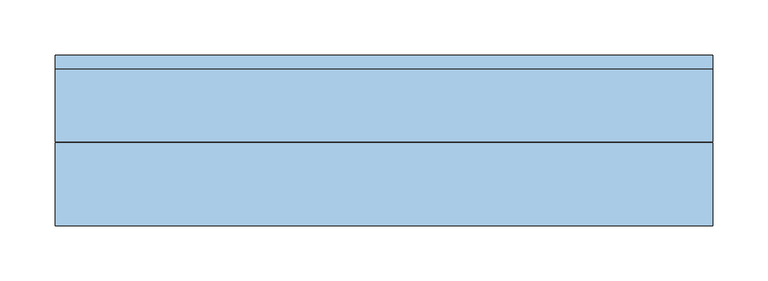
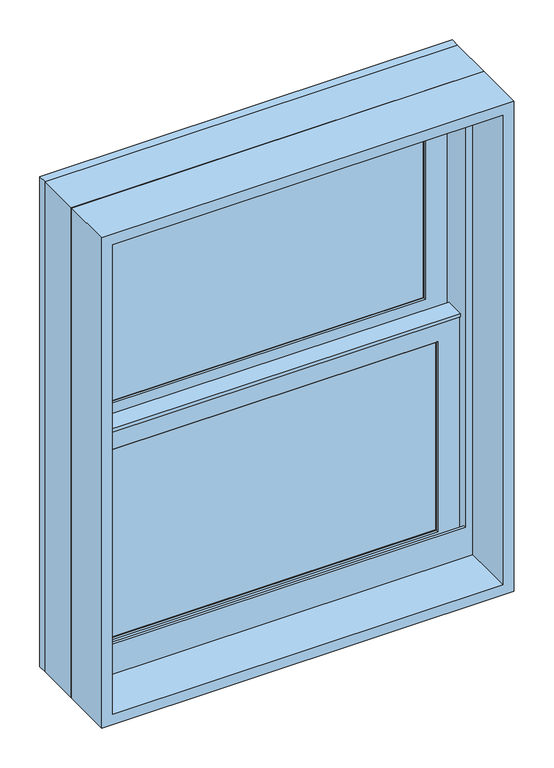
"""IFC4 building model written with IfcOpenShell, lengths in millimetres: window geometry, Window-Double_Hung-Marvin-Essential : ESDH2026."""

import ifcopenshell
import ifcopenshell.guid

model = None  # the IFC model being written
_history = None  # IfcOwnerHistory: only IFC2X3 demands one
_inside = {}  # id of a spatial element -> (the spatial element, [elements in it])
_under = {}  # id of a project, library or spatial element -> (it, [spatial elements below it])
_declared = {}  # id of a project -> (the project, [libraries it declares])
_typed = {}  # id of a type object -> (the type object, [elements of that type])
_made_of = {}  # id of a material, layer set ... -> (it, [elements and type objects made of it])


def new_model(schema):
    """Start an empty IFC model of exactly this schema.

    Asked for "IFC4X3", IfcOpenShell would pick the latest addendum, in which some entities
    have other attributes; the version numbers below select the first issue.
    IFC2X3 requires an IfcOwnerHistory on every rooted entity: one is made here for all.
    """
    global model, _history
    if schema == "IFC4X3":
        model = ifcopenshell.file(schema_version=(4, 3, 0, 0))
    else:
        model = ifcopenshell.file(schema=schema)
    _inside.clear()
    _under.clear()
    _declared.clear()
    _typed.clear()
    _made_of.clear()
    _history = None
    if model.schema == "IFC2X3":
        org = make("IfcOrganization", Name="unknown")
        user = make(
            "IfcPersonAndOrganization",
            ThePerson=make("IfcPerson", FamilyName="unknown"),
            TheOrganization=org,
        )
        app = make(
            "IfcApplication",
            ApplicationDeveloper=org,
            Version="unknown",
            ApplicationFullName="unknown",
            ApplicationIdentifier="unknown",
        )
        _history = make(
            "IfcOwnerHistory",
            OwningUser=user,
            OwningApplication=app,
            ChangeAction="ADDED",
            CreationDate=0,
        )
    return model


def make(cls, **values):
    """One entity of the class cls with the attributes given. An attribute that is None is left unset."""
    return model.create_entity(
        cls, **{name: value for name, value in values.items() if value is not None}
    )


def rooted(cls, **values):
    """An entity with a GlobalId (a new one), such as an element, a storey or a relation."""
    return make(cls, GlobalId=ifcopenshell.guid.new(), OwnerHistory=_history, **values)


def si_unit(unit_type, name, prefix=None):
    """IfcSIUnit, for example si_unit("LENGTHUNIT", "METRE", prefix="MILLI")."""
    return make("IfcSIUnit", UnitType=unit_type, Prefix=prefix, Name=name)


def assignment(units):
    """IfcUnitAssignment: the units of a project."""
    return None if units is None else make("IfcUnitAssignment", Units=units)


def point(xyz):
    """IfcCartesianPoint."""
    return None if xyz is None else make("IfcCartesianPoint", Coordinates=xyz)


def direction(xyz):
    """IfcDirection."""
    return None if xyz is None else make("IfcDirection", DirectionRatios=xyz)


def frame(location, z_axis=None, x_axis=None):
    """IfcAxis2Placement3D, a coordinate frame: its origin and axes. An axis left out is left unset."""
    return make(
        "IfcAxis2Placement3D",
        Location=point(location),
        Axis=direction(z_axis),
        RefDirection=direction(x_axis),
    )


def origin():
    """The frame at (0, 0, 0) with its axes left unset."""
    return frame((0.0, 0.0, 0.0))


def place(relative_to, where):
    """IfcLocalPlacement: puts the frame where relative to a parent placement (None: the world)."""
    return make(
        "IfcLocalPlacement", PlacementRelTo=relative_to, RelativePlacement=where
    )


def context(
    kind, dimensions, precision=None, world=None, true_north=None, identifier=None
):
    """IfcGeometricRepresentationContext, for example the 3D "Model" context."""
    return make(
        "IfcGeometricRepresentationContext",
        ContextIdentifier=identifier,
        ContextType=kind,
        CoordinateSpaceDimension=dimensions,
        Precision=precision,
        WorldCoordinateSystem=world,
        TrueNorth=true_north,
    )


def project(units=None, contexts=None):
    """IfcProject with its units and contexts."""
    return rooted(
        "IfcProject",
        Name="project",
        RepresentationContexts=contexts,
        UnitsInContext=assignment(units),
    )


def spatial(cls, under=None, at=None, **own):
    """A site, building, storey or space (cls), placed at a placement, below another one or the project."""
    s = rooted(cls, ObjectPlacement=at, **own)
    if under is not None:
        _under.setdefault(under.id(), (under, []))[1].append(s)
    return s


def polyline(points):
    """IfcPolyline through the points."""
    return make("IfcPolyline", Points=[point(p) for p in points])


def outline(outer, holes=None, kind="AREA"):
    """IfcArbitraryClosedProfileDef: a profile drawn as a closed curve; with holes, ...WithVoids."""
    if holes is None:
        return make("IfcArbitraryClosedProfileDef", ProfileType=kind, OuterCurve=outer)
    return make(
        "IfcArbitraryProfileDefWithVoids",
        ProfileType=kind,
        OuterCurve=outer,
        InnerCurves=holes,
    )


def extrude(swept, where, along, depth):
    """IfcExtrudedAreaSolid: the profile swept, set in the frame where, extruded along a direction by depth."""
    return make(
        "IfcExtrudedAreaSolid",
        SweptArea=swept,
        Position=where,
        ExtrudedDirection=direction(along),
        Depth=depth,
    )


def faces_of(points, faces, orient=None, outer=None):
    """IfcFace entities. A face is a list of loops; a loop is a list of indices into points, from 0.

    orient and outer hold one flag for each loop. By default every Orientation is true, the
    first loop of a face is its IfcFaceOuterBound and the others are IfcFaceBound.
    """
    made = []
    for i, loops in enumerate(faces):
        bounds = []
        for j, loop in enumerate(loops):
            is_outer = j == 0 if outer is None else outer[i][j]
            bounds.append(
                make(
                    "IfcFaceOuterBound" if is_outer else "IfcFaceBound",
                    Bound=make("IfcPolyLoop", Polygon=[points[k] for k in loop]),
                    Orientation=True if orient is None else orient[i][j],
                )
            )
        made.append(make("IfcFace", Bounds=bounds))
    return made


def faceted_brep(points, faces, orient=None, outer=None, voids=None):
    """IfcFacetedBrep: a solid bounded by flat faces; with voids (closed shells), ...WithVoids."""
    shared = [point(p) for p in points]
    hull = make("IfcClosedShell", CfsFaces=faces_of(shared, faces, orient, outer))
    if voids is None:
        return make("IfcFacetedBrep", Outer=hull)
    return make(
        "IfcFacetedBrepWithVoids",
        Outer=hull,
        Voids=[
            make(cls, CfsFaces=faces_of(shared, fs, o, b)) for cls, fs, o, b in voids
        ],
    )


def shape(context_of_items, identifier, shape_type, items):
    """IfcShapeRepresentation: the items that make up one representation, for example the "Body"."""
    return make(
        "IfcShapeRepresentation",
        ContextOfItems=context_of_items,
        RepresentationIdentifier=identifier,
        RepresentationType=shape_type,
        Items=items,
    )


def source(mapping_origin, context_of_items, identifier, shape_type, items):
    """IfcRepresentationMap: a shape defined once, which mapped items show again and again."""
    return make(
        "IfcRepresentationMap",
        MappingOrigin=mapping_origin,
        MappedRepresentation=shape(context_of_items, identifier, shape_type, items),
    )


def transform(
    local_origin,
    x_axis=None,
    y_axis=None,
    z_axis=None,
    scale=None,
    scale2=None,
    scale3=None,
    uniform=True,
):
    """IfcCartesianTransformationOperator3D, or its non-uniform kind. x_axis, y_axis, z_axis: its Axis1, 2, 3."""
    if uniform:
        return make(
            "IfcCartesianTransformationOperator3D",
            Axis1=direction(x_axis),
            Axis2=direction(y_axis),
            LocalOrigin=point(local_origin),
            Scale=scale,
            Axis3=direction(z_axis),
        )
    return make(
        "IfcCartesianTransformationOperator3DnonUniform",
        Axis1=direction(x_axis),
        Axis2=direction(y_axis),
        LocalOrigin=point(local_origin),
        Scale=scale,
        Axis3=direction(z_axis),
        Scale2=scale2,
        Scale3=scale3,
    )


def mapped(mapping_source, mapping_target):
    """IfcMappedItem: shows the shape of a source again, moved by a transform."""
    return make(
        "IfcMappedItem", MappingSource=mapping_source, MappingTarget=mapping_target
    )


def made_of(thing, what):
    """Note that an element or type object is made of a material, layer set ...; save() writes the relation."""
    if what is not None:
        _made_of.setdefault(what.id(), (what, []))[1].append(thing)
    return thing


def element(
    cls,
    number,
    at=None,
    inside=None,
    cuts=None,
    type_object=None,
    material=None,
    context=None,
    identifier="Body",
    shape_type=None,
    held_by="IfcProductDefinitionShape",
    body=None,
    shapes=None,
    **own,
):
    """One element of the class cls, such as IfcWall. Its Tag is "e" and its number.

    at: its placement. inside: the storey or other place that contains it. cuts: it is an
    opening in that element (IfcRelVoidsElement). A single representation is given by context,
    identifier, shape_type and body (its items); several are given by shapes. held_by: the class
    of the entity that holds the representations. save() writes the other relations.
    """
    e = rooted(cls, Tag="e%d" % number, ObjectPlacement=at, **own)
    if body is not None:
        shapes = [shape(context, identifier, shape_type, body)]
    if shapes is not None:
        e.Representation = make(held_by, Representations=shapes)
    if inside is not None:
        _inside.setdefault(inside.id(), (inside, []))[1].append(e)
    if cuts is not None:
        rooted(
            "IfcRelVoidsElement", RelatingBuildingElement=cuts, RelatedOpeningElement=e
        )
    if type_object is not None:
        _typed.setdefault(type_object.id(), (type_object, []))[1].append(e)
    return made_of(e, material)


def aggregate(whole, parts):
    """IfcRelAggregates: a whole, such as a stair, and the parts it consists of."""
    return rooted("IfcRelAggregates", RelatingObject=whole, RelatedObjects=parts)


def save(model, path):
    """Write the relations noted so far, then the file.

    IfcRelAggregates (storeys below a building ...), IfcRelContainedInSpatialStructure (elements
    in a storey), IfcRelDefinesByType, IfcRelAssociatesMaterial and IfcRelDeclares: one each for
    every whole, place, type object, material and project.
    """
    for whole, parts in _under.values():
        aggregate(whole, parts)
    for where, things in _inside.values():
        rooted(
            "IfcRelContainedInSpatialStructure",
            RelatedElements=things,
            RelatingStructure=where,
        )
    for kind, things in _typed.values():
        rooted("IfcRelDefinesByType", RelatedObjects=things, RelatingType=kind)
    for what, things in _made_of.values():
        rooted("IfcRelAssociatesMaterial", RelatedObjects=things, RelatingMaterial=what)
    for by, libraries in _declared.values():
        rooted("IfcRelDeclares", RelatingContext=by, RelatedDefinitions=libraries)
    model.write(path)


def window_7cff9b80(model_context):
    return source(origin(), model_context, "Body", "SolidModel", [
        extrude(outline(polyline([(89.9583333, 20.6375), (89.9583333, 15.875), (70.9083333, 15.875), (70.9083333, 20.6375), (89.9583333, 20.6375)])), frame((0.0, 0.0, 1746.25), z_axis=(0.0, 0.0, 1.0), x_axis=(1.0, 0.0, 0.0)), (0.0, 0.0, 1.0), 298.45),
        extrude(outline(polyline([(-70.9083333, 20.6375), (-70.9083333, 15.875), (-89.9583333, 15.875), (-89.9583333, 20.6375), (-70.9083333, 20.6375)])), frame((0.0, 0.0, 1746.25), z_axis=(0.0, 0.0, 1.0), x_axis=(1.0, 0.0, 0.0)), (0.0, 0.0, 1.0), 298.45),
        extrude(outline(polyline([(241.3, 20.6375), (241.3, 15.875), (-241.3, 15.875), (-241.3, 20.6375), (241.3, 20.6375)])), frame((0.0, 0.0, 1885.95), z_axis=(0.0, 0.0, 1.0), x_axis=(1.0, 0.0, 0.0)), (0.0, 0.0, 1.0), 19.05),
        extrude(outline(polyline([(-89.9583333, 46.83125), (-89.9583333, 51.59375), (-70.9083333, 51.59375), (-70.9083333, 46.83125), (-89.9583333, 46.83125)])), frame((0.0, 0.0, 2082.8), z_axis=(0.0, 0.0, 1.0), x_axis=(1.0, 0.0, 0.0)), (0.0, 0.0, 1.0), 298.45),
        extrude(outline(polyline([(70.9083333, 46.83125), (70.9083333, 51.59375), (89.9583333, 51.59375), (89.9583333, 46.83125), (70.9083333, 46.83125)])), frame((0.0, 0.0, 2082.8), z_axis=(0.0, 0.0, 1.0), x_axis=(1.0, 0.0, 0.0)), (0.0, 0.0, 1.0), 298.45),
        extrude(outline(polyline([(-241.3, 46.83125), (-241.3, 51.59375), (241.3, 51.59375), (241.3, 46.83125), (-241.3, 46.83125)])), frame((0.0, 0.0, 2222.5), z_axis=(0.0, 0.0, 1.0), x_axis=(1.0, 0.0, 0.0)), (0.0, 0.0, 1.0), 19.05),
        extrude(outline(polyline([(89.9583333, 20.6375), (70.9083333, 20.6375), (70.9083333, 25.4), (89.9583333, 25.4), (89.9583333, 20.6375)])), frame((0.0, 0.0, 1746.25), z_axis=(0.0, 0.0, 1.0), x_axis=(1.0, 0.0, 0.0)), (0.0, 0.0, 1.0), 298.45),
        extrude(outline(polyline([(-70.9083333, 20.6375), (-89.9583333, 20.6375), (-89.9583333, 25.4), (-70.9083333, 25.4), (-70.9083333, 20.6375)])), frame((0.0, 0.0, 1746.25), z_axis=(0.0, 0.0, 1.0), x_axis=(1.0, 0.0, 0.0)), (0.0, 0.0, 1.0), 298.45),
        extrude(outline(polyline([(241.3, 20.6375), (-241.3, 20.6375), (-241.3, 25.4), (241.3, 25.4), (241.3, 20.6375)])), frame((0.0, 0.0, 1885.95), z_axis=(0.0, 0.0, 1.0), x_axis=(1.0, 0.0, 0.0)), (0.0, 0.0, 1.0), 19.05),
        extrude(outline(polyline([(-89.9583333, 56.35625), (-70.9083333, 56.35625), (-70.9083333, 51.59375), (-89.9583333, 51.59375), (-89.9583333, 56.35625)])), frame((0.0, 0.0, 2082.8), z_axis=(0.0, 0.0, 1.0), x_axis=(1.0, 0.0, 0.0)), (0.0, 0.0, 1.0), 298.45),
        extrude(outline(polyline([(70.9083333, 56.35625), (89.9583333, 56.35625), (89.9583333, 51.59375), (70.9083333, 51.59375), (70.9083333, 56.35625)])), frame((0.0, 0.0, 2082.8), z_axis=(0.0, 0.0, 1.0), x_axis=(1.0, 0.0, 0.0)), (0.0, 0.0, 1.0), 298.45),
        extrude(outline(polyline([(-241.3, 56.35625), (241.3, 56.35625), (241.3, 51.59375), (-241.3, 51.59375), (-241.3, 56.35625)])), frame((0.0, 0.0, 2222.5), z_axis=(0.0, 0.0, 1.0), x_axis=(1.0, 0.0, 0.0)), (0.0, 0.0, 1.0), 19.05),
        faceted_brep([(-268.2875, 5.6780605, 2074.7351748), (-268.2875, 5.6780605, 2070.1), (268.2875, 5.6780605, 2070.1), (268.2875, 5.6780605, 2074.7351748), (-268.2875, 34.8118605, 2074.7351748), (268.2875, 34.8118605, 2074.7351748), (268.2875, 34.8118605, 2070.1), (-268.2875, 34.8118605, 2070.1), (-268.2875, 30.1625, 2070.1), (-268.2875, 30.1625, 1719.2625), (-268.2875, 8.9241104, 1719.2625), (-268.2875, 8.9241104, 2070.1), (268.2875, 8.9241104, 2070.1), (268.2875, 30.1625, 2070.1), (268.2875, 8.9241104, 1719.2625), (268.2875, 30.1625, 1719.2625), (-252.4034752, 11.90625, 2055.8034752), (-252.4034752, 30.1625, 2055.8034752), (252.4034752, 30.1625, 2055.8034752), (252.4034752, 11.90625, 2055.8034752), (-235.74375, 10.4662439, 2039.14375), (-235.74375, 11.90625, 2039.14375), (235.74375, 11.90625, 2039.14375), (235.74375, 10.4662439, 2039.14375), (237.2858834, 8.9241104, 2040.6858834), (-237.2858834, 8.9241104, 2040.6858834), (252.4034752, 30.1625, 1735.1465248), (252.4034752, 11.90625, 1735.1465248), (235.74375, 11.90625, 1751.80625), (235.74375, 10.4662439, 1751.80625), (237.2858834, 8.9241104, 1750.2641166), (-252.4034752, 30.1625, 1735.1465248), (-252.4034752, 11.90625, 1735.1465248), (-235.74375, 11.90625, 1751.80625), (-235.74375, 10.4662439, 1751.80625), (-237.2858834, 8.9241104, 1750.2641166)], [[[0, 1, 2, 3]], [[4, 5, 6, 7]], [[1, 0, 4, 7, 8, 9, 10, 11]], [[2, 1, 11, 12]], [[7, 6, 13, 8]], [[3, 2, 12, 14, 15, 13, 6, 5]], [[0, 3, 5, 4]], [[16, 17, 18, 19]], [[20, 21, 22, 23]], [[20, 23, 24, 25]], [[19, 18, 26, 27]], [[23, 22, 28, 29]], [[24, 23, 29, 30]], [[27, 26, 31, 32]], [[29, 28, 33, 34]], [[30, 29, 34, 35]], [[15, 14, 10, 9]], [[15, 9, 8, 13], [18, 17, 31, 26]], [[17, 16, 32, 31]], [[16, 19, 27, 32], [22, 21, 33, 28]], [[21, 20, 34, 33]], [[20, 25, 35, 34]], [[10, 14, 12, 11], [25, 24, 30, 35]]]),
        extrude(outline(polyline([(38.5955581, 2055.8125), (33.5778968, 2055.8125), (33.5778968, 2057.4), (39.9405976, 2057.4), (39.9405976, 2055.8125), (61.515625, 2055.8125), (47.6307501, 2052.4975159), (38.5955581, 2052.4975159), (38.5955581, 2055.8125)])), frame((-268.2875, 0.0, 0.0), z_axis=(1.0, 0.0, 0.0), x_axis=(0.0, 1.0, 0.0)), (0.0, 0.0, 1.0), 536.575),
        faceted_brep([(298.45, 0.0, 1689.1), (298.45, 0.0, 2438.4), (-298.45, 0.0, 2438.4), (-298.45, 0.0, 1689.1), (272.25625, 0.0, 1750.21875), (-272.25625, 0.0, 1750.21875), (-272.25625, 0.0, 2412.20625), (272.25625, 0.0, 2412.20625), (272.25625, 3.96875, 1689.1), (-272.25625, 3.96875, 1689.1), (-272.25625, 3.96875, 1750.21875), (272.25625, 3.96875, 1750.21875), (-298.45, 65.6828125, 1689.1), (-272.25625, 65.6828125, 1689.1), (272.25625, 65.6828125, 1689.1), (298.45, 65.6828125, 1689.1), (-298.45, 65.6828125, 2438.4), (298.45, 65.6828125, 2438.4), (272.25625, 65.6828125, 2412.20625), (-272.25625, 65.6828125, 2412.20625)], [[[0, 1, 2, 3], [4, 5, 6, 7]], [[8, 9, 10, 11]], [[5, 4, 11, 10]], [[0, 3, 12, 13, 9, 8, 14, 15]], [[13, 12, 16, 17, 15, 14, 18, 19]], [[13, 19, 6, 5, 10, 9]], [[7, 6, 19, 18]], [[18, 14, 8, 11, 4, 7]], [[1, 0, 15, 17]], [[2, 1, 17, 16]], [[3, 2, 16, 12]]]),
        faceted_brep([(272.25625, 30.1625, 2063.75), (270.66875, 30.1625, 2063.75), (270.66875, 30.1625, 1713.4544613), (272.25625, 30.1625, 1713.4544613), (-270.66875, 30.1625, 2063.75), (-272.25625, 30.1625, 2063.75), (-272.25625, 30.1625, 1713.4544613), (-270.66875, 30.1625, 1713.4544613), (270.66875, 63.5, 2063.75), (272.25625, 63.5, 2063.75), (272.25625, 63.5, 1706.9743077), (270.66875, 63.5, 1706.9743077), (-272.25625, 63.5, 2063.75), (-270.66875, 63.5, 2063.75), (-270.66875, 63.5, 1706.9743077), (-272.25625, 63.5, 1706.9743077), (283.5108932, 3.96875, 1718.5460105), (283.5108932, 3.96875, 1689.1), (283.5108932, 65.6828125, 1689.1), (283.5108932, 65.6828125, 1706.550012), (-283.5108932, 3.96875, 1689.1), (-283.5108932, 3.96875, 1718.5460105), (-283.5108932, 65.6828125, 1706.550012), (-283.5108932, 65.6828125, 1689.1), (283.5108932, 78.58125, 1704.0428097), (-283.5108932, 78.58125, 1704.0428097), (-281.4971252, 68.2348864, 1706.0539391), (-263.53135, 68.2348864, 1706.0539391), (-263.53135, 65.6828125, 1706.550012), (263.53135, 65.6828125, 1706.550012), (263.53135, 68.2348864, 1706.0539391), (281.4971252, 68.2348864, 1706.0539391), (-298.45, 65.6828125, 1689.1), (-298.45, 78.5948249, 1689.1), (298.45, 78.5948249, 1689.1), (298.45, 65.6828125, 1689.1), (-298.45, 78.58125, 2438.4), (298.45, 78.58125, 2438.4), (283.5108932, 78.58125, 2423.4608932), (-283.5108932, 78.58125, 2423.4608932), (-298.45, 65.6828125, 2438.4), (-281.4971252, 68.2348864, 2421.4471252), (281.4971252, 68.2348864, 2421.4471252), (263.53135, 68.2348864, 2403.48135), (-263.53135, 68.2348864, 2403.48135), (-263.53135, 65.6828125, 2403.48135), (263.53135, 65.6828125, 2403.48135), (298.45, 65.6828125, 2438.4)], [[[0, 1, 2, 3]], [[4, 5, 6, 7]], [[8, 9, 10, 11]], [[12, 13, 14, 15]], [[1, 8, 11, 2]], [[9, 0, 3, 10]], [[1, 0, 9, 8]], [[5, 4, 13, 12]], [[5, 12, 15, 6]], [[13, 4, 7, 14]], [[16, 17, 18, 19]], [[20, 21, 22, 23]], [[24, 25, 26, 27, 28, 22, 21, 16, 19, 29, 30, 31], [3, 2, 11, 10], [7, 6, 15, 14]], [[17, 16, 21, 20]], [[17, 20, 23, 32, 33, 34, 35, 18]], [[34, 33, 36, 37], [25, 24, 38, 39]], [[33, 32, 40, 36]], [[39, 41, 26, 25]], [[41, 42, 31, 30, 43, 44, 27, 26]], [[44, 45, 28, 27]], [[40, 32, 23, 22, 28, 45, 46, 29, 19, 18, 35, 47]], [[36, 40, 47, 37]], [[39, 38, 42, 41]], [[44, 43, 46, 45]], [[34, 37, 47, 35]], [[42, 38, 24, 31]], [[46, 43, 30, 29]]]),
        extrude(outline(polyline([(248.44375, 11.90625), (-248.44375, 11.90625), (-248.44375, 15.08125), (248.44375, 15.08125), (248.44375, 11.90625)])), frame((0.0, 0.0, 1739.10625), z_axis=(0.0, 0.0, 1.0), x_axis=(1.0, 0.0, 0.0)), (0.0, 0.0, 1.0), 312.7375),
        extrude(outline(polyline([(248.44375, 42.8625), (-248.44375, 42.8625), (-248.44375, 46.0375), (248.44375, 46.0375), (248.44375, 42.8625)])), frame((0.0, 0.0, 2075.65625), z_axis=(0.0, 0.0, 1.0), x_axis=(1.0, 0.0, 0.0)), (0.0, 0.0, 1.0), 312.7375),
        faceted_brep([(-235.74375, 31.194477, 2039.14375), (-237.2858834, 32.7366104, 2040.6858834), (237.2858834, 32.7366104, 2040.6858834), (235.74375, 31.194477, 2039.14375), (-235.74375, 30.1625, 2039.14375), (235.74375, 30.1625, 2039.14375), (-268.2875, 32.7366104, 2071.6875), (-268.2875, 30.1625, 2071.6875), (268.2875, 30.1625, 2071.6875), (268.2875, 32.7366104, 2071.6875), (237.2858834, 32.7366104, 1750.2641166), (235.74375, 31.194477, 1751.80625), (235.74375, 30.1625, 1751.80625), (268.2875, 30.1625, 1719.2625), (268.2875, 32.7366104, 1719.2625), (-237.2858834, 32.7366104, 1750.2641166), (-235.74375, 31.194477, 1751.80625), (-235.74375, 30.1625, 1751.80625), (-268.2875, 30.1625, 1719.2625), (-268.2875, 32.7366104, 1719.2625)], [[[0, 1, 2, 3]], [[4, 0, 3, 5]], [[6, 7, 8, 9]], [[3, 2, 10, 11]], [[5, 3, 11, 12]], [[9, 8, 13, 14]], [[11, 10, 15, 16]], [[12, 11, 16, 17]], [[14, 13, 18, 19]], [[9, 14, 19, 6], [1, 15, 10, 2]], [[16, 15, 1, 0]], [[17, 16, 0, 4]], [[7, 18, 13, 8], [5, 12, 17, 4]], [[19, 18, 7, 6]]]),
        faceted_brep([(-252.4034752, 42.8625, 2392.3534752), (-252.4034752, 61.11875, 2392.3534752), (252.4034752, 61.11875, 2392.3534752), (252.4034752, 42.8625, 2392.3534752), (-235.74375, 41.4224939, 2375.69375), (-235.74375, 42.8625, 2375.69375), (235.74375, 42.8625, 2375.69375), (235.74375, 41.4224939, 2375.69375), (-237.2858834, 39.8803604, 2377.2358834), (237.2858834, 39.8803604, 2377.2358834), (-268.2875, 61.11875, 2408.2375), (-268.2875, 39.8803604, 2408.2375), (268.2875, 39.8803604, 2408.2375), (268.2875, 61.11875, 2408.2375), (252.4034752, 61.11875, 2071.6965248), (252.4034752, 42.8625, 2071.6965248), (235.74375, 42.8625, 2088.35625), (235.74375, 41.4224939, 2088.35625), (237.2858834, 39.8803604, 2086.8141166), (268.2875, 39.8803604, 2055.8125), (268.2875, 61.11875, 2055.8125), (-252.4034752, 61.11875, 2071.6965248), (-252.4034752, 42.8625, 2071.6965248), (-235.74375, 42.8625, 2088.35625), (-235.74375, 41.4224939, 2088.35625), (-237.2858834, 39.8803604, 2086.8141166), (-268.2875, 39.8803604, 2055.8125), (-268.2875, 61.11875, 2055.8125)], [[[0, 1, 2, 3]], [[4, 5, 6, 7]], [[8, 4, 7, 9]], [[10, 11, 12, 13]], [[3, 2, 14, 15]], [[7, 6, 16, 17]], [[9, 7, 17, 18]], [[13, 12, 19, 20]], [[15, 14, 21, 22]], [[17, 16, 23, 24]], [[18, 17, 24, 25]], [[20, 19, 26, 27]], [[13, 20, 27, 10], [1, 21, 14, 2]], [[22, 21, 1, 0]], [[3, 15, 22, 0], [5, 23, 16, 6]], [[24, 23, 5, 4]], [[25, 24, 4, 8]], [[11, 26, 19, 12], [9, 18, 25, 8]], [[27, 26, 11, 10]]]),
        faceted_brep([(-268.2875, 61.11875, 2055.8125), (-268.2875, 63.6928604, 2055.8125), (268.2875, 63.6928604, 2055.8125), (268.2875, 61.11875, 2055.8125), (-235.74375, 62.150727, 2088.35625), (-235.74375, 61.11875, 2088.35625), (235.74375, 61.11875, 2088.35625), (235.74375, 62.150727, 2088.35625), (-237.2858834, 63.6928604, 2086.8141166), (237.2858834, 63.6928604, 2086.8141166), (268.2875, 63.6928604, 2408.2375), (268.2875, 61.11875, 2408.2375), (235.74375, 61.11875, 2375.69375), (235.74375, 62.150727, 2375.69375), (237.2858834, 63.6928604, 2377.2358834), (-268.2875, 63.6928604, 2408.2375), (-268.2875, 61.11875, 2408.2375), (-235.74375, 61.11875, 2375.69375), (-235.74375, 62.150727, 2375.69375), (-237.2858834, 63.6928604, 2377.2358834)], [[[0, 1, 2, 3]], [[4, 5, 6, 7]], [[8, 4, 7, 9]], [[3, 2, 10, 11]], [[7, 6, 12, 13]], [[9, 7, 13, 14]], [[11, 10, 15, 16]], [[13, 12, 17, 18]], [[14, 13, 18, 19]], [[16, 15, 1, 0]], [[3, 11, 16, 0], [5, 17, 12, 6]], [[18, 17, 5, 4]], [[19, 18, 4, 8]], [[1, 15, 10, 2], [9, 14, 19, 8]]]),
        extrude(outline(polyline([(248.44375, 26.19375), (-248.44375, 26.19375), (-248.44375, 30.1625), (248.44375, 30.1625), (248.44375, 26.19375)])), frame((0.0, 0.0, 1739.10625), z_axis=(0.0, 0.0, 1.0), x_axis=(1.0, 0.0, 0.0)), (0.0, 0.0, 1.0), 312.7375),
        extrude(outline(polyline([(248.44375, 57.15), (-248.44375, 57.15), (-248.44375, 61.11875), (248.44375, 61.11875), (248.44375, 57.15)])), frame((0.0, 0.0, 2075.65625), z_axis=(0.0, 0.0, 1.0), x_axis=(1.0, 0.0, 0.0)), (0.0, 0.0, 1.0), 312.7375),
        extrude(outline(polyline([(2438.4, 298.45), (2438.4, -298.45), (1689.1, -298.45), (1689.1, 298.45), (2438.4, 298.45)]), holes=[polyline([(2422.525, 282.575), (1704.975, 282.575), (1704.975, -282.575), (2422.525, -282.575), (2422.525, 282.575)])]), frame((0.0, -76.2, 0.0), z_axis=(0.0, 1.0, 0.0), x_axis=(0.0, 0.0, 1.0)), (0.0, 0.0, 1.0), 75.40625),
    ])


if __name__ == "__main__":
    model = new_model("IFC4")
    model_context = context("Model", 3, world=origin())
    ifc_project = project(units=[si_unit("LENGTHUNIT", "METRE", prefix="MILLI")], contexts=[model_context])
    site = spatial("IfcSite", under=ifc_project)
    building = spatial("IfcBuilding", under=site)
    placement = place(None, origin())
    window_shape = window_7cff9b80(model_context)
    element("IfcWindow", 1, ObjectType="Window-Double_Hung-Marvin-Essential : ESDH2026", at=placement, inside=building, context=model_context, shape_type="MappedRepresentation", body=[
        mapped(window_shape, transform((0.0, 0.0, 0.0), x_axis=(1.0, 0.0, 0.0), y_axis=(0.0, 1.0, 0.0), z_axis=(0.0, 0.0, 1.0))),
    ])
    save(model, "model.ifc")

# Revit data of these elements
# Type "Window-Double_Hung-Marvin-Essential : ESDH2026"
#   Type Mark = "27"
#   Window Type = "Essential Double Hung"
#   Product data url = "https://bimobject.com/marvin-windows-and-doors/product/marvin-dhwau"
#   Product Guid = "c4a96547-874c-4385-91dc-a058adc19d98"
#   Frame = "All Ultrex"
#   Egress Window = "No"
#   URL = "www.marvin.com"
#   Model = "ESDH2026"
#   Manufacturer = "Marvin Windows and Doors"
#   Label Egress = ""
#   Glass Type = "IG Low E II with Argon"
#   Design Pressure = "DP50"
#   Description = "2430 DBHG"
#   Analytic Construction = "<None>"
#   Prairie Corner Width = 0' - 4"
#   Prairie Corner Height = 0' - 4"
#   Egress Width = 1' - 8 9/16"
#   Egress Height = 0' - 10 27/128"
#   Rough Width = 2' - 0"
#   Rough Height = 2' - 6"
#   Nominal Width = 2' - 0"
#   Nominal Height = 2' - 6"
#   Inset to Installation Flange [instance default] = 0' - 1"
#   Height = 2' - 5 1/2"
#   Egress Area = 1.45807 SF
#   Default Head Height = 8' - 0"
#   Width = 1' - 11 1/2"
#   Daylight Area = 2.9165 SF
#   DLO Width = 1' - 6 9/16"
#   DLO Height = 0' - 11 5/16"
#   Muntins Top Sash = yes
#   Lites Wide Top Sash = 3
#   Lites Wide Bottom Sash = 3
#   Lites High Top Sash = 2
#   Lites High Bottom Sash = 2
#   Lite Cut Prairie 9 = no
#   Lite Cut HV Grid = yes
#   Muntins Bottom Sash = yes
#   Label Visibility = no
#   Jamb Extension Visibility = yes
#   Edition number = 1
#   Interior Material = Ultrex-Marvin-Stonewhite
#   Glazing Material = Glass-Marvin-IG Low E II with Argon
#   Cladding Material = Ultrex-Marvin-Pebblegray
#   Wall Closure = (empty or 0)
#   Assembly Code = ""
# Element 1 (IfcWindow, "Window-Double_Hung-Marvin-Essential : ESDH2026")
#   Materials on its faces: "Ultrex-Marvin-Pebblegray", "Ultrex-Marvin-Stonewhite", "Glass-Marvin-IG Low E II with Argon"
# Materials
#   "Ultrex-Marvin-Stonewhite": class "Paint", colour RGB 250 251 245, transparency 0
#   "Glass-Marvin-IG Low E II with Argon": class "Glass", colour RGB 0 128 192, transparency 0.85
#   "Ultrex-Marvin-Pebblegray": class "Paint", colour RGB 189 185 173, transparency 0
